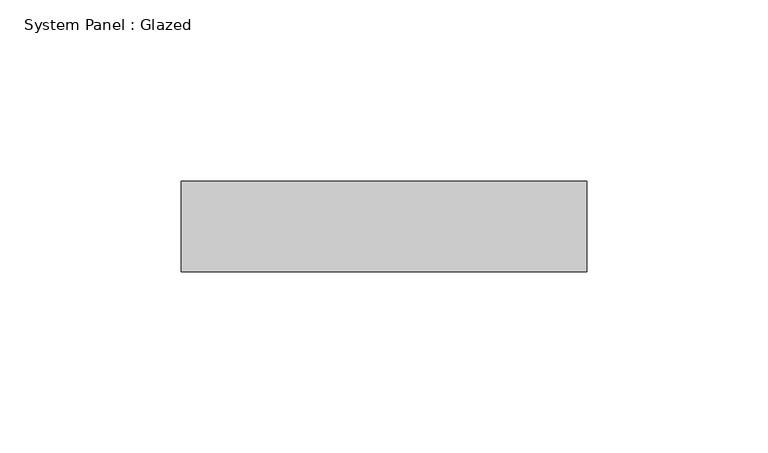
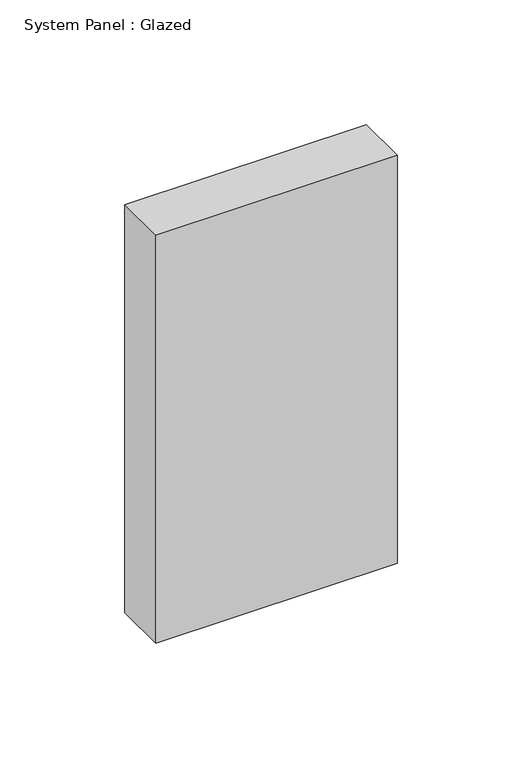
"""IFC4 building model written with IfcOpenShell, lengths in millimetres: plate geometry, System Panel : Glazed."""

from ifc_helpers import new_model, si_unit, origin, origin_with_axes, place, context, project, spatial, polyline, outline, extrude, source, transform, mapped, element, save


def system_panel_glazed_1aaa8be2(model_context):
    return source(origin(), model_context, "Body", "SweptSolid", [
        extrude(outline(polyline([(56.0139357, 24.5), (-56.0139357, 24.5), (-56.0139357, 49.5), (56.0139357, 49.5), (56.0139357, 24.5)])), origin_with_axes(), (0.0, 0.0, 1.0), 200.0),
    ])


if __name__ == "__main__":
    model = new_model("IFC4")
    model_context = context("Model", 3, world=origin())
    ifc_project = project(units=[si_unit("LENGTHUNIT", "METRE", prefix="MILLI")], contexts=[model_context])
    site = spatial("IfcSite", under=ifc_project)
    building = spatial("IfcBuilding", under=site)
    placement = place(None, origin())
    system_panel_glazed_shape = system_panel_glazed_1aaa8be2(model_context)
    element("IfcPlate", 1, ObjectType="System Panel : Glazed", at=placement, inside=building, context=model_context, shape_type="MappedRepresentation", body=[
        mapped(system_panel_glazed_shape, transform((0.0, 0.0, 0.0), x_axis=(1.0, 0.0, 0.0), y_axis=(0.0, 1.0, 0.0), z_axis=(0.0, 0.0, 1.0))),
    ])
    save(model, "model.ifc")

# Revit data of these elements
# Element 1 (IfcPlate, "System Panel : Glazed")
#   Materials on its faces: "Glass"
# Materials
#   "Glass": class "Glass", colour RGB 218 227 224, transparency 0.85, Description = "Soda Lime Glass", Cost = 0
